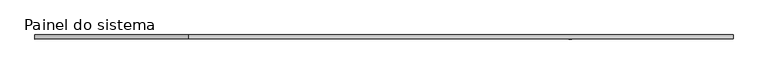
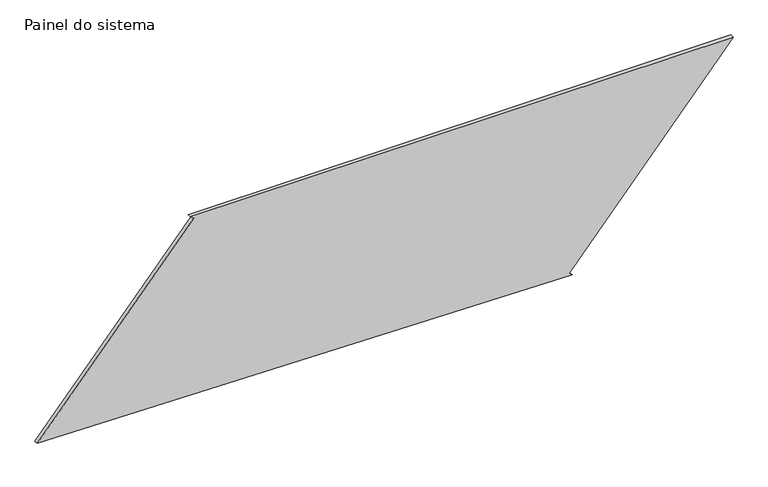
"""IFC4 building model written with IfcOpenShell, lengths in millimetres: plate geometry, Painel do sistema : Envidraçado."""

from ifc_helpers import new_model, si_unit, frame, origin, place, context, project, spatial, polyline, outline, extrude, source, transform, mapped, element, save


def painel_do_sistema_585cbc86(model_context):
    return source(origin(), model_context, "Body", "SweptSolid", [
        extrude(outline(polyline([(0.0, 1153.9307918), (16.2242617, 1134.9104518), (1202.5662853, 2146.8546937), (1202.5662853, -1201.7039358), (1186.3420236, -1182.6835959), (56.0063352, -2146.8546937), (0.0, 1153.9307918)])), frame((0.0, 24.5, 0.0), z_axis=(0.0, 1.0, 0.0), x_axis=(0.0, 0.0, 1.0)), (0.0, 0.0, 1.0), 25.0),
    ])


if __name__ == "__main__":
    model = new_model("IFC4")
    model_context = context("Model", 3, world=origin())
    ifc_project = project(units=[si_unit("LENGTHUNIT", "METRE", prefix="MILLI")], contexts=[model_context])
    site = spatial("IfcSite", under=ifc_project)
    building = spatial("IfcBuilding", under=site)
    placement = place(None, origin())
    painel_do_sistema_shape = painel_do_sistema_585cbc86(model_context)
    element("IfcPlate", 1, ObjectType="Painel do sistema : Envidraçado", at=placement, inside=building, context=model_context, shape_type="MappedRepresentation", body=[
        mapped(painel_do_sistema_shape, transform((0.0, 0.0, 0.0), x_axis=(1.0, 0.0, 0.0), y_axis=(0.0, 1.0, 0.0), z_axis=(0.0, 0.0, 1.0))),
    ])
    save(model, "model.ifc")

# Revit data of these elements
# Type "Painel do sistema : Envidraçado"
#   Construction Type Id = "GSP4R"
#   Analytic Construction = "Vidraça única Pilkington 1/8 pol"
#   Visual Light Transmittance = 0.9
#   Solar Heat Gain Coefficient = 0.86
#   Heat Transfer Coefficient (U) = 6.7069 W/(m²·K)
# Element 1 (IfcPlate, "Painel do sistema : Envidraçado")
#   Materials on its faces: "Vidro"
# Materials
#   "Vidro": class "Vidro", colour RGB 0 128 192, transparency 0.9, Description = "Vidro de sílica", Cost = 0
